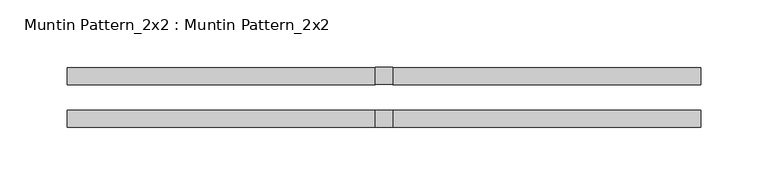
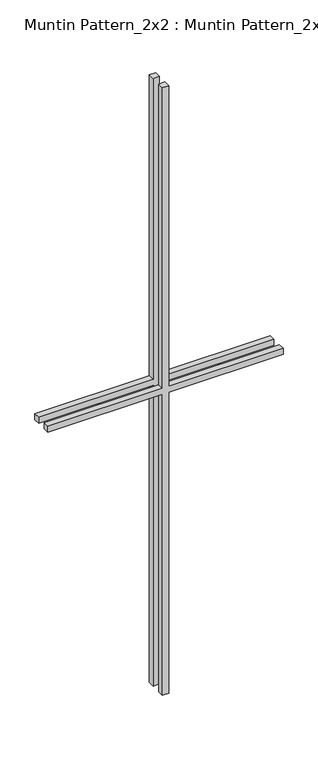
"""IFC4 building model written with IfcOpenShell, lengths in millimetres: proxy geometry, Muntin Pattern_2x2 : Muntin Pattern_2x2."""

import ifcopenshell
import ifcopenshell.guid

model = None  # the IFC model being written
_history = None  # IfcOwnerHistory: only IFC2X3 demands one
_inside = {}  # id of a spatial element -> (the spatial element, [elements in it])
_under = {}  # id of a project, library or spatial element -> (it, [spatial elements below it])
_declared = {}  # id of a project -> (the project, [libraries it declares])
_typed = {}  # id of a type object -> (the type object, [elements of that type])
_made_of = {}  # id of a material, layer set ... -> (it, [elements and type objects made of it])


def new_model(schema):
    """Start an empty IFC model of exactly this schema.

    Asked for "IFC4X3", IfcOpenShell would pick the latest addendum, in which some entities
    have other attributes; the version numbers below select the first issue.
    IFC2X3 requires an IfcOwnerHistory on every rooted entity: one is made here for all.
    """
    global model, _history
    if schema == "IFC4X3":
        model = ifcopenshell.file(schema_version=(4, 3, 0, 0))
    else:
        model = ifcopenshell.file(schema=schema)
    _inside.clear()
    _under.clear()
    _declared.clear()
    _typed.clear()
    _made_of.clear()
    _history = None
    if model.schema == "IFC2X3":
        org = make("IfcOrganization", Name="unknown")
        user = make(
            "IfcPersonAndOrganization",
            ThePerson=make("IfcPerson", FamilyName="unknown"),
            TheOrganization=org,
        )
        app = make(
            "IfcApplication",
            ApplicationDeveloper=org,
            Version="unknown",
            ApplicationFullName="unknown",
            ApplicationIdentifier="unknown",
        )
        _history = make(
            "IfcOwnerHistory",
            OwningUser=user,
            OwningApplication=app,
            ChangeAction="ADDED",
            CreationDate=0,
        )
    return model


def make(cls, **values):
    """One entity of the class cls with the attributes given. An attribute that is None is left unset."""
    return model.create_entity(
        cls, **{name: value for name, value in values.items() if value is not None}
    )


def rooted(cls, **values):
    """An entity with a GlobalId (a new one), such as an element, a storey or a relation."""
    return make(cls, GlobalId=ifcopenshell.guid.new(), OwnerHistory=_history, **values)


def si_unit(unit_type, name, prefix=None):
    """IfcSIUnit, for example si_unit("LENGTHUNIT", "METRE", prefix="MILLI")."""
    return make("IfcSIUnit", UnitType=unit_type, Prefix=prefix, Name=name)


def assignment(units):
    """IfcUnitAssignment: the units of a project."""
    return None if units is None else make("IfcUnitAssignment", Units=units)


def point(xyz):
    """IfcCartesianPoint."""
    return None if xyz is None else make("IfcCartesianPoint", Coordinates=xyz)


def direction(xyz):
    """IfcDirection."""
    return None if xyz is None else make("IfcDirection", DirectionRatios=xyz)


def frame(location, z_axis=None, x_axis=None):
    """IfcAxis2Placement3D, a coordinate frame: its origin and axes. An axis left out is left unset."""
    return make(
        "IfcAxis2Placement3D",
        Location=point(location),
        Axis=direction(z_axis),
        RefDirection=direction(x_axis),
    )


def origin():
    """The frame at (0, 0, 0) with its axes left unset."""
    return frame((0.0, 0.0, 0.0))


def place(relative_to, where):
    """IfcLocalPlacement: puts the frame where relative to a parent placement (None: the world)."""
    return make(
        "IfcLocalPlacement", PlacementRelTo=relative_to, RelativePlacement=where
    )


def context(
    kind, dimensions, precision=None, world=None, true_north=None, identifier=None
):
    """IfcGeometricRepresentationContext, for example the 3D "Model" context."""
    return make(
        "IfcGeometricRepresentationContext",
        ContextIdentifier=identifier,
        ContextType=kind,
        CoordinateSpaceDimension=dimensions,
        Precision=precision,
        WorldCoordinateSystem=world,
        TrueNorth=true_north,
    )


def project(units=None, contexts=None):
    """IfcProject with its units and contexts."""
    return rooted(
        "IfcProject",
        Name="project",
        RepresentationContexts=contexts,
        UnitsInContext=assignment(units),
    )


def spatial(cls, under=None, at=None, **own):
    """A site, building, storey or space (cls), placed at a placement, below another one or the project."""
    s = rooted(cls, ObjectPlacement=at, **own)
    if under is not None:
        _under.setdefault(under.id(), (under, []))[1].append(s)
    return s


def polyline(points):
    """IfcPolyline through the points."""
    return make("IfcPolyline", Points=[point(p) for p in points])


def outline(outer, holes=None, kind="AREA"):
    """IfcArbitraryClosedProfileDef: a profile drawn as a closed curve; with holes, ...WithVoids."""
    if holes is None:
        return make("IfcArbitraryClosedProfileDef", ProfileType=kind, OuterCurve=outer)
    return make(
        "IfcArbitraryProfileDefWithVoids",
        ProfileType=kind,
        OuterCurve=outer,
        InnerCurves=holes,
    )


def extrude(swept, where, along, depth):
    """IfcExtrudedAreaSolid: the profile swept, set in the frame where, extruded along a direction by depth."""
    return make(
        "IfcExtrudedAreaSolid",
        SweptArea=swept,
        Position=where,
        ExtrudedDirection=direction(along),
        Depth=depth,
    )


def shape(context_of_items, identifier, shape_type, items):
    """IfcShapeRepresentation: the items that make up one representation, for example the "Body"."""
    return make(
        "IfcShapeRepresentation",
        ContextOfItems=context_of_items,
        RepresentationIdentifier=identifier,
        RepresentationType=shape_type,
        Items=items,
    )


def source(mapping_origin, context_of_items, identifier, shape_type, items):
    """IfcRepresentationMap: a shape defined once, which mapped items show again and again."""
    return make(
        "IfcRepresentationMap",
        MappingOrigin=mapping_origin,
        MappedRepresentation=shape(context_of_items, identifier, shape_type, items),
    )


def transform(
    local_origin,
    x_axis=None,
    y_axis=None,
    z_axis=None,
    scale=None,
    scale2=None,
    scale3=None,
    uniform=True,
):
    """IfcCartesianTransformationOperator3D, or its non-uniform kind. x_axis, y_axis, z_axis: its Axis1, 2, 3."""
    if uniform:
        return make(
            "IfcCartesianTransformationOperator3D",
            Axis1=direction(x_axis),
            Axis2=direction(y_axis),
            LocalOrigin=point(local_origin),
            Scale=scale,
            Axis3=direction(z_axis),
        )
    return make(
        "IfcCartesianTransformationOperator3DnonUniform",
        Axis1=direction(x_axis),
        Axis2=direction(y_axis),
        LocalOrigin=point(local_origin),
        Scale=scale,
        Axis3=direction(z_axis),
        Scale2=scale2,
        Scale3=scale3,
    )


def mapped(mapping_source, mapping_target):
    """IfcMappedItem: shows the shape of a source again, moved by a transform."""
    return make(
        "IfcMappedItem", MappingSource=mapping_source, MappingTarget=mapping_target
    )


def made_of(thing, what):
    """Note that an element or type object is made of a material, layer set ...; save() writes the relation."""
    if what is not None:
        _made_of.setdefault(what.id(), (what, []))[1].append(thing)
    return thing


def element(
    cls,
    number,
    at=None,
    inside=None,
    cuts=None,
    type_object=None,
    material=None,
    context=None,
    identifier="Body",
    shape_type=None,
    held_by="IfcProductDefinitionShape",
    body=None,
    shapes=None,
    **own,
):
    """One element of the class cls, such as IfcWall. Its Tag is "e" and its number.

    at: its placement. inside: the storey or other place that contains it. cuts: it is an
    opening in that element (IfcRelVoidsElement). A single representation is given by context,
    identifier, shape_type and body (its items); several are given by shapes. held_by: the class
    of the entity that holds the representations. save() writes the other relations.
    """
    e = rooted(cls, Tag="e%d" % number, ObjectPlacement=at, **own)
    if body is not None:
        shapes = [shape(context, identifier, shape_type, body)]
    if shapes is not None:
        e.Representation = make(held_by, Representations=shapes)
    if inside is not None:
        _inside.setdefault(inside.id(), (inside, []))[1].append(e)
    if cuts is not None:
        rooted(
            "IfcRelVoidsElement", RelatingBuildingElement=cuts, RelatedOpeningElement=e
        )
    if type_object is not None:
        _typed.setdefault(type_object.id(), (type_object, []))[1].append(e)
    return made_of(e, material)


def aggregate(whole, parts):
    """IfcRelAggregates: a whole, such as a stair, and the parts it consists of."""
    return rooted("IfcRelAggregates", RelatingObject=whole, RelatedObjects=parts)


def save(model, path):
    """Write the relations noted so far, then the file.

    IfcRelAggregates (storeys below a building ...), IfcRelContainedInSpatialStructure (elements
    in a storey), IfcRelDefinesByType, IfcRelAssociatesMaterial and IfcRelDeclares: one each for
    every whole, place, type object, material and project.
    """
    for whole, parts in _under.values():
        aggregate(whole, parts)
    for where, things in _inside.values():
        rooted(
            "IfcRelContainedInSpatialStructure",
            RelatedElements=things,
            RelatingStructure=where,
        )
    for kind, things in _typed.values():
        rooted("IfcRelDefinesByType", RelatedObjects=things, RelatingType=kind)
    for what, things in _made_of.values():
        rooted("IfcRelAssociatesMaterial", RelatedObjects=things, RelatingMaterial=what)
    for by, libraries in _declared.values():
        rooted("IfcRelDeclares", RelatingContext=by, RelatedDefinitions=libraries)
    model.write(path)


def muntin_pattern_2x2_muntin_pattern_2x2_5bc79d00(model_context):
    return source(origin(), model_context, "Body", "SweptSolid", [
        extrude(outline(polyline([(647.7, -6.35), (647.7, -234.95), (635.0, -234.95), (635.0, -6.35), (0.0, -6.35), (0.0, 6.35), (635.0, 6.35), (635.0, 234.95), (647.7, 234.95), (647.7, 6.35), (1282.7, 6.35), (1282.7, -6.35), (647.7, -6.35)])), frame((0.0, -22.225, 0.0), z_axis=(0.0, 1.0, 0.0), x_axis=(0.0, 0.0, 1.0)), (0.0, 0.0, 1.0), 12.7),
        extrude(outline(polyline([(647.7, -6.35), (647.7, -234.95), (635.0, -234.95), (635.0, -6.35), (0.0, -6.35), (0.0, 6.35), (635.0, 6.35), (635.0, 234.95), (647.7, 234.95), (647.7, 6.35), (1282.7, 6.35), (1282.7, -6.35), (647.7, -6.35)])), frame((0.0, 9.525, 0.0), z_axis=(0.0, 1.0, 0.0), x_axis=(0.0, 0.0, 1.0)), (0.0, 0.0, 1.0), 12.7),
    ])


if __name__ == "__main__":
    model = new_model("IFC4")
    model_context = context("Model", 3, world=origin())
    ifc_project = project(units=[si_unit("LENGTHUNIT", "METRE", prefix="MILLI")], contexts=[model_context])
    site = spatial("IfcSite", under=ifc_project)
    building = spatial("IfcBuilding", under=site)
    placement = place(None, origin())
    muntin_pattern_2x2_muntin_pattern_2x2_shape = muntin_pattern_2x2_muntin_pattern_2x2_5bc79d00(model_context)
    element("IfcBuildingElementProxy", 1, Name="Muntin Pattern_2x2 : Muntin Pattern_2x2", ObjectType="Muntin Pattern_2x2 : Muntin Pattern_2x2", at=placement, inside=building, context=model_context, shape_type="MappedRepresentation", body=[
        mapped(muntin_pattern_2x2_muntin_pattern_2x2_shape, transform((0.0, 0.0, 0.0), x_axis=(1.0, 0.0, 0.0), y_axis=(0.0, 1.0, 0.0), z_axis=(0.0, 0.0, 1.0))),
    ])
    save(model, "model.ifc")

# Revit data of these elements
# Type "Muntin Pattern_2x2 : Muntin Pattern_2x2"
#   Width [instance default] = 4' - 0"
#   Thickness = 0' - 0 1/2"
#   Height [instance default] = 4' - 0"
#   Distance = 0' - 0 3/4"
#   Interior Material [instance default] = none
#   Exterior Material [instance default] = none
#   Default Elevation = 0
# Element 1 (IfcBuildingElementProxy, "Muntin Pattern_2x2 : Muntin Pattern_2x2")
#   Width = 1' - 6 1/2"
#   Height = 4' - 2 1/2"
#   Interior Material = Wood - Stained
#   Exterior Material = Clad - White
#   Materials on its faces: "Clad - White", "Wood - Stained"
# Materials
#   "Clad - White": class "Wood", colour RGB 242 242 238, transparency 0, Cost = 0
#   "Wood - Stained": class "Wood", colour RGB 224 178 126, transparency 0, Cost = 0
